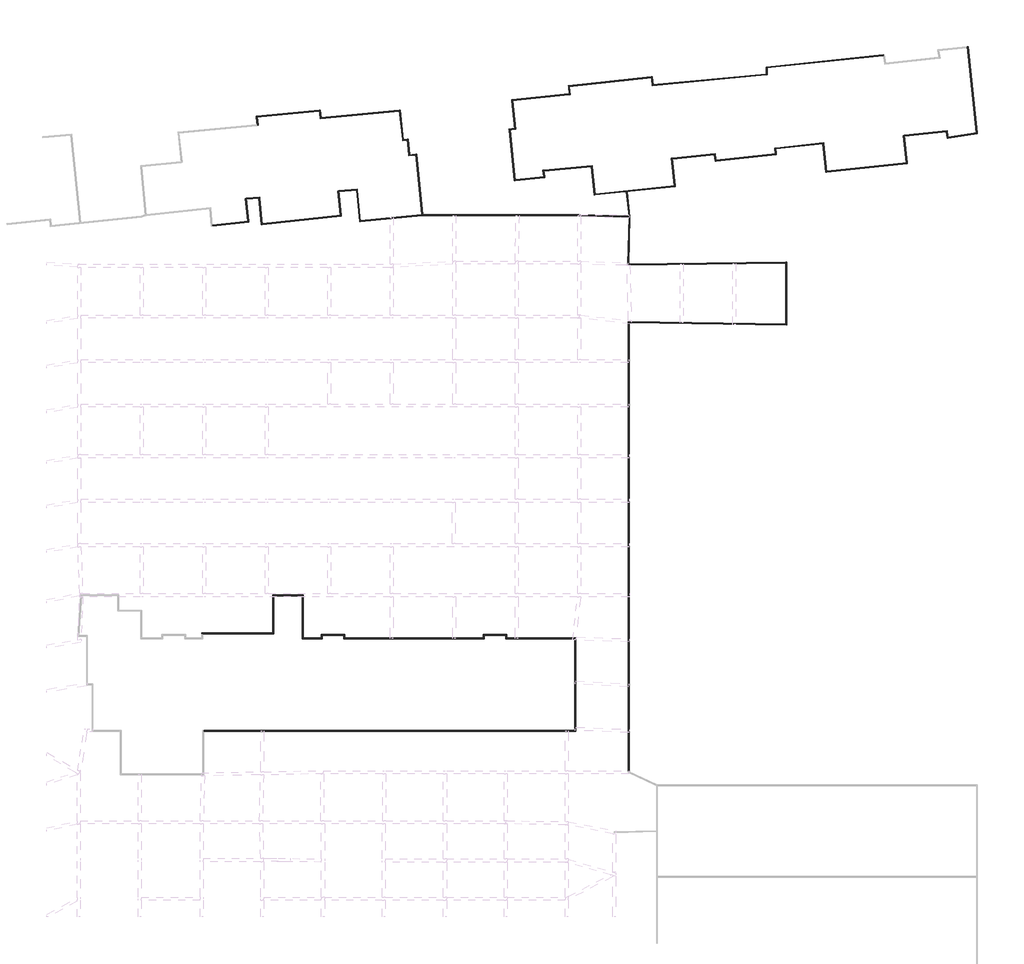
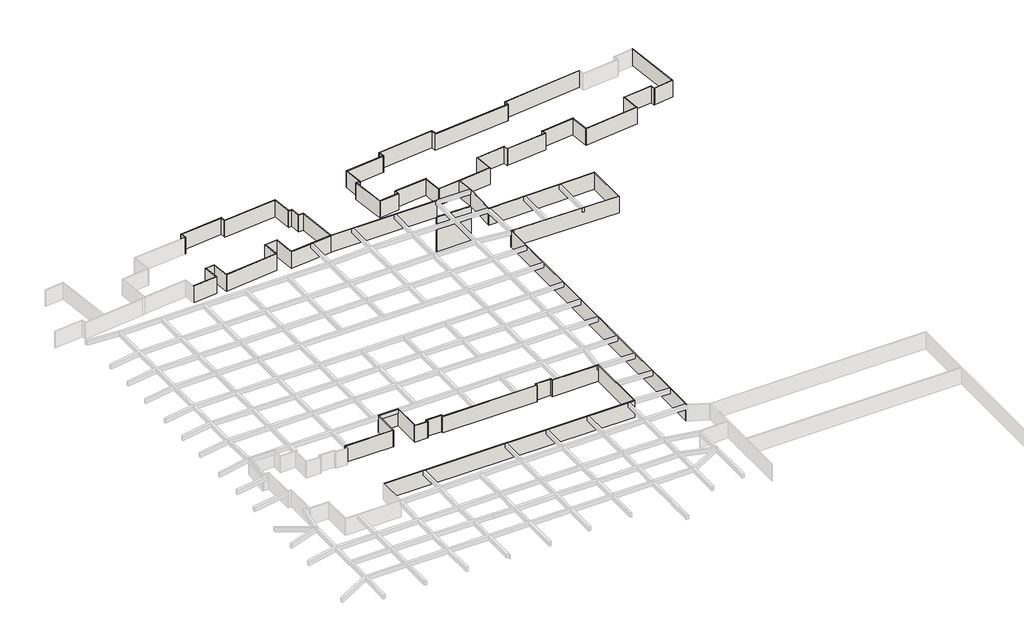
# One storey, part 7 of 20: 70 walls.
"""IFC4 building model written with IfcOpenShell, lengths in millimetres."""

from ifc_helpers import new_model, si_unit, frame, origin, origin_with_axes, place, context, project, spatial, polyline, outline, extrude, faceted_brep, element, save

model = new_model("IFC4")

# Units and contexts
model_context = context("Model", 3, world=origin())
ifc_project = project(units=[si_unit("LENGTHUNIT", "METRE", prefix="MILLI")], contexts=[model_context])

# Site, building, storey
site = spatial("IfcSite", under=ifc_project)
building = spatial("IfcBuilding", under=site)
storey = spatial("IfcBuildingStorey", under=building, Name="户型图", Elevation=0.0)

# Walls
placement = place(None, origin())
element("IfcWall", 1, ObjectType="所有墙体", at=placement, inside=storey, context=model_context, shape_type="SweptSolid", body=[
    extrude(outline(polyline([(179359.7688515, 185330.8967461), (179359.7688515, 127752.6972626), (179239.7688515, 127808.6541816), (179239.7688515, 185332.6895961), (179359.7688515, 185330.8967461)])), origin_with_axes(), (0.0, 0.0, 1.0), 3300.0),
])
element("IfcWall", 2, ObjectType="所有墙体", at=placement, inside=storey, context=model_context, shape_type="Brep", body=[
    faceted_brep([(179239.7688515, 185332.6895961, 0.0), (179359.7688515, 185330.8967461, 0.0), (199560.0, 185029.0968789, 0.0), (199560.0, 185029.0968789, 3300.0), (179359.7688515, 185330.8967461, 3300.0), (179239.7688515, 185332.6895961, 3300.0), (179239.7688515, 185452.7029883, 0.0), (179239.7688515, 185452.7029883, 3300.0), (199560.0, 185149.1102711, 3300.0), (199560.0, 185149.1102711, 0.0)], [[[0, 1, 2, 3, 4, 5]], [[6, 7, 8, 9]], [[2, 1, 0, 6, 9]], [[5, 4, 3, 8, 7]], [[0, 5, 7, 6]], [[3, 2, 9, 8]]]),
])
element("IfcWall", 3, ObjectType="所有墙体", at=placement, inside=storey, context=model_context, shape_type="Brep", body=[
    faceted_brep([(199560.0, 185149.1102711, 0.0), (199560.0, 193050.6703703, 0.0), (199560.0, 193050.6703703, 3300.0), (199560.0, 185149.1102711, 3300.0), (199440.0, 185150.9031211, 0.0), (199440.0, 185150.9031211, 3300.0), (199440.0, 192929.3296297, 3300.0), (199440.0, 193049.3370369, 3300.0), (199440.0, 193049.3370369, 0.0), (199440.0, 192929.3296297, 0.0)], [[[0, 1, 2, 3]], [[4, 5, 6, 7, 8, 9]], [[1, 0, 4, 9, 8]], [[3, 2, 7, 6, 5]], [[2, 1, 8, 7]], [[0, 3, 5, 4]]]),
])
element("IfcWall", 4, ObjectType="所有墙体", at=placement, inside=storey, context=model_context, shape_type="Brep", body=[
    faceted_brep([(199440.0, 193049.3370369, 0.0), (179311.5042041, 192825.6870836, 0.0), (179191.4355527, 192824.3529875, 0.0), (179191.4355527, 192824.3529875, 3300.0), (179311.5042041, 192825.6870836, 3300.0), (199440.0, 193049.3370369, 3300.0), (199440.0, 192929.3296297, 0.0), (199440.0, 192929.3296297, 3300.0), (179188.4957959, 192704.3129164, 3300.0), (179188.4957959, 192704.3129164, 0.0)], [[[0, 1, 2, 3, 4, 5]], [[6, 7, 8, 9]], [[2, 1, 0, 6, 9]], [[5, 4, 3, 8, 7]], [[0, 5, 7, 6]], [[3, 2, 9, 8]]]),
])
element("IfcWall", 5, ObjectType="所有墙体", at=placement, inside=storey, context=model_context, shape_type="SweptSolid", body=[
    extrude(outline(polyline([(179460.0770452, 198892.4114303), (179311.5042041, 192825.6870836), (179191.4355527, 192824.3529875), (179339.9229548, 198887.5885697), (179460.0770452, 198892.4114303)])), origin_with_axes(), (0.0, 0.0, 1.0), 3300.0),
])
element("IfcWall", 6, ObjectType="所有墙体", at=placement, inside=storey, context=model_context, shape_type="SweptSolid", body=[
    extrude(outline(polyline([(179120.9990927, 202118.5226488), (179460.0770452, 198892.4114303), (179339.9229548, 198887.5885697), (179001.6564653, 202105.9792332), (179120.9990927, 202118.5226488)])), origin_with_axes(), (0.0, 0.0, 1.0), 3300.0),
])
element("IfcWall", 7, ObjectType="所有墙体", at=placement, inside=storey, context=model_context, shape_type="Brep", body=[
    faceted_brep([(175009.081088, 201686.3426514, 0.0), (179001.6564653, 202105.9792332, 0.0), (179120.9990927, 202118.5226488, 0.0), (185275.013613, 202765.3356388, 0.0), (185275.013613, 202765.3356388, 3300.0), (179120.9990927, 202118.5226488, 3300.0), (179001.6564653, 202105.9792332, 3300.0), (175009.081088, 201686.3426514, 3300.0), (174996.5376724, 201805.6852789, 0.0), (174996.5376724, 201805.6852789, 3300.0), (185143.1275699, 202872.1348506, 3300.0), (185262.4701974, 202884.6782662, 3300.0), (185262.4701974, 202884.6782662, 0.0), (185143.1275699, 202872.1348506, 0.0)], [[[0, 1, 2, 3, 4, 5, 6, 7]], [[8, 9, 10, 11, 12, 13]], [[3, 2, 1, 0, 8, 13, 12]], [[7, 6, 5, 4, 11, 10, 9]], [[4, 3, 12, 11]], [[0, 7, 9, 8]]]),
])
element("IfcWall", 8, ObjectType="所有墙体", at=placement, inside=storey, context=model_context, shape_type="Brep", body=[
    faceted_brep([(185262.4701974, 202884.6782662, 0.0), (184906.1157461, 206275.1643906, 0.0), (184893.5723305, 206394.5070181, 0.0), (184893.5723305, 206394.5070181, 3300.0), (184906.1157461, 206275.1643906, 3300.0), (185262.4701974, 202884.6782662, 3300.0), (185143.1275699, 202872.1348506, 0.0), (185143.1275699, 202872.1348506, 3300.0), (184774.229703, 206381.9636025, 3300.0), (184774.229703, 206381.9636025, 0.0)], [[[0, 1, 2, 3, 4, 5]], [[6, 7, 8, 9]], [[2, 1, 0, 6, 9]], [[5, 4, 3, 8, 7]], [[0, 5, 7, 6]], [[3, 2, 9, 8]]]),
])
element("IfcWall", 9, ObjectType="所有墙体", at=placement, inside=storey, context=model_context, shape_type="Brep", body=[
    faceted_brep([(184906.1157461, 206275.1643906, 0.0), (190280.8750728, 206840.0743594, 0.0), (190400.2177003, 206852.617775, 0.0), (190400.2177003, 206852.617775, 3300.0), (190280.8750728, 206840.0743594, 3300.0), (184906.1157461, 206275.1643906, 3300.0), (184893.5723305, 206394.5070181, 0.0), (184893.5723305, 206394.5070181, 3300.0), (190387.6742847, 206971.9604024, 3300.0), (190387.6742847, 206971.9604024, 0.0)], [[[0, 1, 2, 3, 4, 5]], [[6, 7, 8, 9]], [[2, 1, 0, 6, 9]], [[5, 4, 3, 8, 7]], [[0, 5, 7, 6]], [[3, 2, 9, 8]]]),
])
element("IfcWall", 10, ObjectType="所有墙体", at=placement, inside=storey, context=model_context, shape_type="Brep", body=[
    faceted_brep([(190280.8750728, 206840.0743594, 0.0), (190368.4732423, 206006.6334497, 0.0), (190368.4732423, 206006.6334497, 3300.0), (190280.8750728, 206840.0743594, 3300.0), (190400.2177003, 206852.617775, 0.0), (190400.2177003, 206852.617775, 3300.0), (190475.2724541, 206138.5194927, 3300.0), (190487.8158697, 206019.1768653, 3300.0), (190487.8158697, 206019.1768653, 0.0), (190475.2724541, 206138.5194927, 0.0)], [[[0, 1, 2, 3]], [[4, 5, 6, 7, 8, 9]], [[1, 0, 4, 9, 8]], [[3, 2, 7, 6, 5]], [[0, 3, 5, 4]], [[2, 1, 8, 7]]]),
])
element("IfcWall", 11, ObjectType="所有墙体", at=placement, inside=storey, context=model_context, shape_type="Brep", body=[
    faceted_brep([(190487.8158697, 206019.1768653, 0.0), (198188.6858964, 206828.5709203, 0.0), (198188.6858964, 206828.5709203, 3300.0), (190487.8158697, 206019.1768653, 3300.0), (190475.2724541, 206138.5194927, 0.0), (190475.2724541, 206138.5194927, 3300.0), (198056.7998534, 206935.3701322, 3300.0), (198176.1424808, 206947.9135478, 3300.0), (198176.1424808, 206947.9135478, 0.0), (198056.7998534, 206935.3701322, 0.0)], [[[0, 1, 2, 3]], [[4, 5, 6, 7, 8, 9]], [[1, 0, 4, 9, 8]], [[3, 2, 7, 6, 5]], [[0, 3, 5, 4]], [[2, 1, 8, 7]]]),
])
element("IfcWall", 12, ObjectType="所有墙体", at=placement, inside=storey, context=model_context, shape_type="Brep", body=[
    faceted_brep([(198176.1424808, 206947.9135478, 0.0), (198110.6347971, 207571.1775256, 0.0), (198098.0913815, 207690.520153, 0.0), (198098.0913815, 207690.520153, 3300.0), (198110.6347971, 207571.1775256, 3300.0), (198176.1424808, 206947.9135478, 3300.0), (198056.7998534, 206935.3701322, 0.0), (198056.7998534, 206935.3701322, 3300.0), (197978.748754, 207677.9767374, 3300.0), (197978.748754, 207677.9767374, 0.0)], [[[0, 1, 2, 3, 4, 5]], [[6, 7, 8, 9]], [[2, 1, 0, 6, 9]], [[5, 4, 3, 8, 7]], [[0, 5, 7, 6]], [[3, 2, 9, 8]]]),
])
element("IfcWall", 13, ObjectType="所有墙体", at=placement, inside=storey, context=model_context, shape_type="Brep", body=[
    faceted_brep([(198110.6347971, 207571.1775256, 0.0), (204161.7596128, 208207.1763718, 0.0), (204281.1022402, 208219.7197874, 0.0), (204281.1022402, 208219.7197874, 3300.0), (204161.7596128, 208207.1763718, 3300.0), (198110.6347971, 207571.1775256, 3300.0), (198098.0913815, 207690.520153, 0.0), (198098.0913815, 207690.520153, 3300.0), (204268.5588247, 208339.0624149, 3300.0), (204268.5588247, 208339.0624149, 0.0)], [[[0, 1, 2, 3, 4, 5]], [[6, 7, 8, 9]], [[2, 1, 0, 6, 9]], [[5, 4, 3, 8, 7]], [[0, 5, 7, 6]], [[3, 2, 9, 8]]]),
])
element("IfcWall", 14, ObjectType="所有墙体", at=placement, inside=storey, context=model_context, shape_type="Brep", body=[
    faceted_brep([(204161.7596128, 208207.1763718, 0.0), (204542.5743461, 204583.9662099, 0.0), (204542.5743461, 204583.9662099, 3300.0), (204161.7596128, 208207.1763718, 3300.0), (204281.1022402, 208219.7197874, 0.0), (204281.1022402, 208219.7197874, 3300.0), (204649.3735579, 204715.8522529, 3300.0), (204661.9169735, 204596.5096255, 3300.0), (204661.9169735, 204596.5096255, 0.0), (204649.3735579, 204715.8522529, 0.0)], [[[0, 1, 2, 3]], [[4, 5, 6, 7, 8, 9]], [[1, 0, 4, 9, 8]], [[3, 2, 7, 6, 5]], [[0, 3, 5, 4]], [[2, 1, 8, 7]]]),
])
element("IfcWall", 15, ObjectType="所有墙体", at=placement, inside=storey, context=model_context, shape_type="Brep", body=[
    faceted_brep([(204661.9169735, 204596.5096255, 0.0), (214978.0466758, 205680.7785487, 0.0), (214978.0466758, 205680.7785487, 3300.0), (204661.9169735, 204596.5096255, 3300.0), (204649.3735579, 204715.8522529, 0.0), (204649.3735579, 204715.8522529, 3300.0), (214846.1606327, 205787.5777606, 3300.0), (214965.5032602, 205800.1211762, 3300.0), (214965.5032602, 205800.1211762, 0.0), (214846.1606327, 205787.5777606, 0.0)], [[[0, 1, 2, 3]], [[4, 5, 6, 7, 8, 9]], [[1, 0, 4, 9, 8]], [[3, 2, 7, 6, 5]], [[0, 3, 5, 4]], [[2, 1, 8, 7]]]),
])
element("IfcWall", 16, ObjectType="所有墙体", at=placement, inside=storey, context=model_context, shape_type="Brep", body=[
    faceted_brep([(214965.5032602, 205800.1211762, 0.0), (214609.1847922, 209190.2649423, 0.0), (214596.6413766, 209309.6075698, 0.0), (214596.6413766, 209309.6075698, 3300.0), (214609.1847922, 209190.2649423, 3300.0), (214965.5032602, 205800.1211762, 3300.0), (214846.1606327, 205787.5777606, 0.0), (214846.1606327, 205787.5777606, 3300.0), (214477.2987492, 209297.0641542, 3300.0), (214477.2987492, 209297.0641542, 0.0)], [[[0, 1, 2, 3, 4, 5]], [[6, 7, 8, 9]], [[2, 1, 0, 6, 9]], [[5, 4, 3, 8, 7]], [[0, 5, 7, 6]], [[3, 2, 9, 8]]]),
])
element("IfcWall", 17, ObjectType="所有墙体", at=placement, inside=storey, context=model_context, shape_type="Brep", body=[
    faceted_brep([(214609.1847922, 209190.2649423, 0.0), (219982.9732093, 209755.0728644, 0.0), (220102.3158367, 209767.61628, 0.0), (220102.3158367, 209767.61628, 3300.0), (219982.9732093, 209755.0728644, 3300.0), (214609.1847922, 209190.2649423, 3300.0), (214596.6413766, 209309.6075698, 0.0), (214596.6413766, 209309.6075698, 3300.0), (220089.7724211, 209886.9589074, 3300.0), (220089.7724211, 209886.9589074, 0.0)], [[[0, 1, 2, 3, 4, 5]], [[6, 7, 8, 9]], [[2, 1, 0, 6, 9]], [[5, 4, 3, 8, 7]], [[0, 5, 7, 6]], [[3, 2, 9, 8]]]),
])
element("IfcWall", 18, ObjectType="所有墙体", at=placement, inside=storey, context=model_context, shape_type="Brep", body=[
    faceted_brep([(219982.9732093, 209755.0728644, 0.0), (220070.8035215, 208919.4232641, 0.0), (220070.8035215, 208919.4232641, 3300.0), (219982.9732093, 209755.0728644, 3300.0), (220102.3158367, 209767.61628, 0.0), (220102.3158367, 209767.61628, 3300.0), (220176.9281469, 209057.7275686, 3300.0), (220189.4887764, 208938.2211617, 3300.0), (220189.4887764, 208938.2211617, 0.0), (220176.9281469, 209057.7275686, 0.0)], [[[0, 1, 2, 3]], [[4, 5, 6, 7, 8, 9]], [[1, 0, 4, 9, 8]], [[3, 2, 7, 6, 5]], [[0, 3, 5, 4]], [[2, 1, 8, 7]]]),
])
element("IfcWall", 19, ObjectType="所有墙体", at=placement, inside=storey, context=model_context, shape_type="Brep", body=[
    faceted_brep([(220189.4887764, 208938.2211617, 0.0), (223943.6146969, 209532.8162946, 0.0), (223943.6146969, 209532.8162946, 3300.0), (220189.4887764, 208938.2211617, 3300.0), (220176.9281469, 209057.7275686, 0.0), (220176.9281469, 209057.7275686, 3300.0), (223812.3688125, 209633.5248037, 3300.0), (223931.0540674, 209652.3227014, 3300.0), (223931.0540674, 209652.3227014, 0.0), (223812.3688125, 209633.5248037, 0.0)], [[[0, 1, 2, 3]], [[4, 5, 6, 7, 8, 9]], [[1, 0, 4, 9, 8]], [[3, 2, 7, 6, 5]], [[0, 3, 5, 4]], [[2, 1, 8, 7]]]),
])
element("IfcWall", 20, ObjectType="所有墙体", at=placement, inside=storey, context=model_context, shape_type="Brep", body=[
    faceted_brep([(223931.0540674, 209652.3227014, 0.0), (222771.1254183, 220688.3066092, 0.0), (222771.1254183, 220688.3066092, 3300.0), (223931.0540674, 209652.3227014, 3300.0), (223812.3688125, 209633.5248037, 0.0), (223812.3688125, 209633.5248037, 3300.0), (222664.3262065, 220556.4205662, 3300.0), (222651.7827909, 220675.7631937, 3300.0), (222651.7827909, 220675.7631937, 0.0), (222664.3262065, 220556.4205662, 0.0)], [[[0, 1, 2, 3]], [[4, 5, 6, 7, 8, 9]], [[1, 0, 4, 9, 8]], [[3, 2, 7, 6, 5]], [[0, 3, 5, 4]], [[2, 1, 8, 7]]]),
])
element("IfcWall", 21, ObjectType="所有墙体", at=placement, inside=storey, context=model_context, shape_type="Brep", body=[
    faceted_brep([(211896.3577151, 219645.7354926, 0.0), (196892.6398704, 218068.7812024, 0.0), (196892.6398704, 218068.7812024, 3300.0), (211896.3577151, 219645.7354926, 3300.0), (211915.1556128, 219527.0502378, 0.0), (211915.1556128, 219527.0502378, 3300.0), (197012.6398704, 217960.7327171, 3300.0), (196892.6398704, 217948.1202089, 3300.0), (196892.6398704, 217948.1202089, 0.0), (197012.6398704, 217960.7327171, 0.0)], [[[0, 1, 2, 3]], [[4, 5, 6, 7, 8, 9]], [[1, 0, 4, 9, 8]], [[3, 2, 7, 6, 5]], [[0, 3, 5, 4]], [[2, 1, 8, 7]]]),
])
element("IfcWall", 22, ObjectType="所有墙体", at=placement, inside=storey, context=model_context, shape_type="Brep", body=[
    faceted_brep([(196892.6398704, 217948.1202089, 0.0), (196892.6398704, 217169.3650376, 0.0), (196892.6398704, 217048.832647, 0.0), (196892.6398704, 217048.832647, 3300.0), (196892.6398704, 217169.3650376, 3300.0), (196892.6398704, 217948.1202089, 3300.0), (197012.6398704, 217960.7327171, 0.0), (197012.6398704, 217960.7327171, 3300.0), (197012.6398704, 217060.148882, 3300.0), (197012.6398704, 217060.148882, 0.0)], [[[0, 1, 2, 3, 4, 5]], [[6, 7, 8, 9]], [[2, 1, 0, 6, 9]], [[5, 4, 3, 8, 7]], [[0, 5, 7, 6]], [[3, 2, 9, 8]]]),
])
element("IfcWall", 23, ObjectType="所有墙体", at=placement, inside=storey, context=model_context, shape_type="Brep", body=[
    faceted_brep([(196892.6398704, 217169.3650376, 0.0), (182438.466331, 215806.308175, 0.0), (182318.9895359, 215795.0412793, 0.0), (182318.9895359, 215795.0412793, 3300.0), (182438.466331, 215806.308175, 3300.0), (196892.6398704, 217169.3650376, 3300.0), (196892.6398704, 217048.832647, 0.0), (196892.6398704, 217048.832647, 3300.0), (182331.533669, 215675.691825, 3300.0), (182331.533669, 215675.691825, 0.0)], [[[0, 1, 2, 3, 4, 5]], [[6, 7, 8, 9]], [[2, 1, 0, 6, 9]], [[5, 4, 3, 8, 7]], [[0, 5, 7, 6]], [[3, 2, 9, 8]]]),
])
element("IfcWall", 24, ObjectType="所有墙体", at=placement, inside=storey, context=model_context, shape_type="Brep", body=[
    faceted_brep([(182438.466331, 215806.308175, 0.0), (182333.8711427, 216801.4649169, 0.0), (182333.8711427, 216801.4649169, 3300.0), (182438.466331, 215806.308175, 3300.0), (182318.9895359, 215795.0412793, 0.0), (182318.9895359, 215795.0412793, 3300.0), (182227.0719308, 216669.5788739, 3300.0), (182214.5285152, 216788.9215013, 3300.0), (182214.5285152, 216788.9215013, 0.0), (182227.0719308, 216669.5788739, 0.0)], [[[0, 1, 2, 3]], [[4, 5, 6, 7, 8, 9]], [[1, 0, 4, 9, 8]], [[3, 2, 7, 6, 5]], [[0, 3, 5, 4]], [[2, 1, 8, 7]]]),
])
element("IfcWall", 25, ObjectType="所有墙体", at=placement, inside=storey, context=model_context, shape_type="Brep", body=[
    faceted_brep([(182214.5285152, 216788.9215013, 0.0), (171581.168922, 215671.3103729, 0.0), (171581.168922, 215671.3103729, 3300.0), (182214.5285152, 216788.9215013, 3300.0), (182227.0719308, 216669.5788739, 0.0), (182227.0719308, 216669.5788739, 3300.0), (171713.054965, 215564.5111611, 3300.0), (171593.7123376, 215551.9677455, 3300.0), (171593.7123376, 215551.9677455, 0.0), (171713.054965, 215564.5111611, 0.0)], [[[0, 1, 2, 3]], [[4, 5, 6, 7, 8, 9]], [[1, 0, 4, 9, 8]], [[3, 2, 7, 6, 5]], [[0, 3, 5, 4]], [[2, 1, 8, 7]]]),
])
element("IfcWall", 26, ObjectType="所有墙体", at=placement, inside=storey, context=model_context, shape_type="Brep", body=[
    faceted_brep([(171593.7123376, 215551.9677455, 0.0), (171690.7043845, 214629.150062, 0.0), (171703.2478001, 214509.8074345, 0.0), (171703.2478001, 214509.8074345, 3300.0), (171690.7043845, 214629.150062, 3300.0), (171593.7123376, 215551.9677455, 3300.0), (171713.054965, 215564.5111611, 0.0), (171713.054965, 215564.5111611, 3300.0), (171822.5904275, 214522.3508501, 3300.0), (171822.5904275, 214522.3508501, 0.0)], [[[0, 1, 2, 3, 4, 5]], [[6, 7, 8, 9]], [[2, 1, 0, 6, 9]], [[5, 4, 3, 8, 7]], [[0, 5, 7, 6]], [[3, 2, 9, 8]]]),
])
element("IfcWall", 27, ObjectType="所有墙体", at=placement, inside=storey, context=model_context, shape_type="Brep", body=[
    faceted_brep([(171690.7043845, 214629.150062, 0.0), (164300.405986, 213852.3984004, 0.0), (164300.405986, 213852.3984004, 3300.0), (171690.7043845, 214629.150062, 3300.0), (171703.2478001, 214509.8074345, 0.0), (171703.2478001, 214509.8074345, 3300.0), (164432.2920291, 213745.5991886, 3300.0), (164312.9494016, 213733.055773, 3300.0), (164312.9494016, 213733.055773, 0.0), (164432.2920291, 213745.5991886, 0.0)], [[[0, 1, 2, 3]], [[4, 5, 6, 7, 8, 9]], [[1, 0, 4, 9, 8]], [[3, 2, 7, 6, 5]], [[0, 3, 5, 4]], [[2, 1, 8, 7]]]),
])
element("IfcWall", 28, ObjectType="所有墙体", at=placement, inside=storey, context=model_context, shape_type="Brep", body=[
    faceted_brep([(164312.9494016, 213733.055773, 0.0), (164684.8655737, 210194.5097657, 0.0), (164697.4089893, 210075.1671382, 0.0), (164697.4089893, 210075.1671382, 3300.0), (164684.8655737, 210194.5097657, 3300.0), (164312.9494016, 213733.055773, 3300.0), (164432.2920291, 213745.5991886, 0.0), (164432.2920291, 213745.5991886, 3300.0), (164816.7516167, 210087.7105538, 3300.0), (164816.7516167, 210087.7105538, 0.0)], [[[0, 1, 2, 3, 4, 5]], [[6, 7, 8, 9]], [[2, 1, 0, 6, 9]], [[5, 4, 3, 8, 7]], [[0, 5, 7, 6]], [[3, 2, 9, 8]]]),
])
element("IfcWall", 29, ObjectType="所有墙体", at=placement, inside=storey, context=model_context, shape_type="Brep", body=[
    faceted_brep([(164684.8655737, 210194.5097657, 0.0), (163969.8374545, 210119.357282, 0.0), (163969.8374545, 210119.357282, 3300.0), (164684.8655737, 210194.5097657, 3300.0), (164697.4089893, 210075.1671382, 0.0), (164697.4089893, 210075.1671382, 3300.0), (164101.7234975, 210012.5580702, 3300.0), (163982.3808701, 210000.0146546, 3300.0), (163982.3808701, 210000.0146546, 0.0), (164101.7234975, 210012.5580702, 0.0)], [[[0, 1, 2, 3]], [[4, 5, 6, 7, 8, 9]], [[1, 0, 4, 9, 8]], [[3, 2, 7, 6, 5]], [[0, 3, 5, 4]], [[2, 1, 8, 7]]]),
])
element("IfcWall", 30, ObjectType="所有墙体", at=placement, inside=storey, context=model_context, shape_type="Brep", body=[
    faceted_brep([(163982.3808701, 210000.0146546, 0.0), (164664.446564, 203510.5930613, 0.0), (164664.446564, 203510.5930613, 3300.0), (163982.3808701, 210000.0146546, 3300.0), (164101.7234975, 210012.5580702, 0.0), (164101.7234975, 210012.5580702, 3300.0), (164771.2457758, 203642.4791043, 3300.0), (164783.7891914, 203523.1364769, 3300.0), (164783.7891914, 203523.1364769, 0.0), (164771.2457758, 203642.4791043, 0.0)], [[[0, 1, 2, 3]], [[4, 5, 6, 7, 8, 9]], [[1, 0, 4, 9, 8]], [[3, 2, 7, 6, 5]], [[0, 3, 5, 4]], [[2, 1, 8, 7]]]),
])
element("IfcWall", 31, ObjectType="所有墙体", at=placement, inside=storey, context=model_context, shape_type="Brep", body=[
    faceted_brep([(164783.7891914, 203523.1364769, 0.0), (168536.3797426, 203917.549637, 0.0), (168536.3797426, 203917.549637, 3300.0), (164783.7891914, 203523.1364769, 3300.0), (164771.2457758, 203642.4791043, 0.0), (164771.2457758, 203642.4791043, 3300.0), (168404.4936996, 204024.3488489, 3300.0), (168523.836327, 204036.8922645, 3300.0), (168523.836327, 204036.8922645, 0.0), (168404.4936996, 204024.3488489, 0.0)], [[[0, 1, 2, 3]], [[4, 5, 6, 7, 8, 9]], [[1, 0, 4, 9, 8]], [[3, 2, 7, 6, 5]], [[0, 3, 5, 4]], [[2, 1, 8, 7]]]),
])
element("IfcWall", 32, ObjectType="所有墙体", at=placement, inside=storey, context=model_context, shape_type="Brep", body=[
    faceted_brep([(168523.836327, 204036.8922645, 0.0), (168453.0383983, 204710.4895608, 0.0), (168440.4942645, 204829.8390215, 0.0), (168440.4942645, 204829.8390215, 3300.0), (168453.0383983, 204710.4895608, 3300.0), (168523.836327, 204036.8922645, 3300.0), (168404.4936996, 204024.3488489, 0.0), (168404.4936996, 204024.3488489, 3300.0), (168321.0174056, 204818.5727331, 3300.0), (168321.0174056, 204818.5727331, 0.0)], [[[0, 1, 2, 3, 4, 5]], [[6, 7, 8, 9]], [[2, 1, 0, 6, 9]], [[5, 4, 3, 8, 7]], [[0, 5, 7, 6]], [[3, 2, 9, 8]]]),
])
element("IfcWall", 33, ObjectType="所有墙体", at=placement, inside=storey, context=model_context, shape_type="Brep", body=[
    faceted_brep([(168453.0383983, 204710.4895608, 0.0), (174510.5336374, 205281.6921254, 0.0), (174630.0104964, 205292.9584138, 0.0), (174630.0104964, 205292.9584138, 3300.0), (174510.5336374, 205281.6921254, 3300.0), (168453.0383983, 204710.4895608, 3300.0), (168440.4942645, 204829.8390215, 0.0), (168440.4942645, 204829.8390215, 3300.0), (174617.4663626, 205412.3078746, 3300.0), (174617.4663626, 205412.3078746, 0.0)], [[[0, 1, 2, 3, 4, 5]], [[6, 7, 8, 9]], [[2, 1, 0, 6, 9]], [[5, 4, 3, 8, 7]], [[0, 5, 7, 6]], [[3, 2, 9, 8]]]),
])
element("IfcWall", 34, ObjectType="所有墙体", at=placement, inside=storey, context=model_context, shape_type="Brep", body=[
    faceted_brep([(174510.5336374, 205281.6921254, 0.0), (174889.7384605, 201673.7992358, 0.0), (174889.7384605, 201673.7992358, 3300.0), (174510.5336374, 205281.6921254, 3300.0), (174630.0104964, 205292.9584138, 0.0), (174630.0104964, 205292.9584138, 3300.0), (174996.5376724, 201805.6852789, 3300.0), (175009.081088, 201686.3426514, 3300.0), (175009.081088, 201686.3426514, 0.0), (174996.5376724, 201805.6852789, 0.0)], [[[0, 1, 2, 3]], [[4, 5, 6, 7, 8, 9]], [[1, 0, 4, 9, 8]], [[3, 2, 7, 6, 5]], [[0, 3, 5, 4]], [[2, 1, 8, 7]]]),
])
element("IfcWall", 35, ObjectType="所有墙体", at=placement, inside=storey, context=model_context, shape_type="Brep", body=[
    faceted_brep([(152798.3916431, 199007.0, 0.0), (172953.0, 199007.0, 0.0), (172953.0, 199007.0, 3300.0), (152798.3916431, 199007.0, 3300.0), (152787.0760242, 199127.0, 0.0), (152787.0760242, 199127.0, 3300.0), (152907.6083569, 199127.0, 3300.0), (172953.0, 199127.0, 3300.0), (172953.0, 199127.0, 0.0), (152907.6083569, 199127.0, 0.0)], [[[0, 1, 2, 3]], [[4, 5, 6, 7, 8, 9]], [[1, 0, 4, 9, 8]], [[2, 1, 8, 7]], [[3, 2, 7, 6, 5]], [[0, 3, 5, 4]]]),
])
element("IfcWall", 36, ObjectType="所有墙体", at=placement, inside=storey, context=model_context, shape_type="Brep", body=[
    faceted_brep([(172953.0, 199127.0, 0.0), (152907.6083569, 199127.0, 0.0), (152787.0760242, 199127.0, 0.0), (152787.0760242, 199127.0, 3300.0), (152907.6083569, 199127.0, 3300.0), (172953.0, 199127.0, 3300.0), (172953.0, 199007.0, 0.0), (172953.0, 199007.0, 3300.0), (152798.3916431, 199007.0, 3300.0), (152798.3916431, 199007.0, 0.0)], [[[0, 1, 2, 3, 4, 5]], [[6, 7, 8, 9]], [[2, 1, 0, 6, 9]], [[5, 4, 3, 8, 7]], [[0, 5, 7, 6]], [[3, 2, 9, 8]]]),
])
element("IfcWall", 37, ObjectType="所有墙体", at=placement, inside=storey, context=model_context, shape_type="Brep", body=[
    faceted_brep([(152907.6083569, 199127.0, 0.0), (152174.8353707, 206897.9190224, 0.0), (152174.8353707, 206897.9190224, 3300.0), (152907.6083569, 199127.0, 3300.0), (152787.0760242, 199127.0, 0.0), (152787.0760242, 199127.0, 3300.0), (152066.6309957, 206767.1833607, 3300.0), (152055.3653523, 206886.6533791, 3300.0), (152055.3653523, 206886.6533791, 0.0), (152066.6309957, 206767.1833607, 0.0)], [[[0, 1, 2, 3]], [[4, 5, 6, 7, 8, 9]], [[1, 0, 4, 9, 8]], [[3, 2, 7, 6, 5]], [[0, 3, 5, 4]], [[2, 1, 8, 7]]]),
])
element("IfcWall", 38, ObjectType="所有墙体", at=placement, inside=storey, context=model_context, shape_type="Brep", body=[
    faceted_brep([(152055.3653523, 206886.6533791, 0.0), (151247.154558, 206810.4416677, 0.0), (151127.6776991, 206799.1753794, 0.0), (151127.6776991, 206799.1753794, 3300.0), (151247.154558, 206810.4416677, 3300.0), (152055.3653523, 206886.6533791, 3300.0), (152066.6309957, 206767.1833607, 0.0), (152066.6309957, 206767.1833607, 3300.0), (151140.2218329, 206679.8259186, 3300.0), (151140.2218329, 206679.8259186, 0.0)], [[[0, 1, 2, 3, 4, 5]], [[6, 7, 8, 9]], [[2, 1, 0, 6, 9]], [[5, 4, 3, 8, 7]], [[0, 5, 7, 6]], [[3, 2, 9, 8]]]),
])
element("IfcWall", 39, ObjectType="所有墙体", at=placement, inside=storey, context=model_context, shape_type="Brep", body=[
    faceted_brep([(151247.154558, 206810.4416677, 0.0), (151038.0308748, 208800.1206054, 0.0), (151038.0308748, 208800.1206054, 3300.0), (151247.154558, 206810.4416677, 3300.0), (151127.6776991, 206799.1753794, 0.0), (151127.6776991, 206799.1753794, 3300.0), (150931.231663, 208668.2345624, 3300.0), (150918.6882474, 208787.5771898, 3300.0), (150918.6882474, 208787.5771898, 0.0), (150931.231663, 208668.2345624, 0.0)], [[[0, 1, 2, 3]], [[4, 5, 6, 7, 8, 9]], [[1, 0, 4, 9, 8]], [[3, 2, 7, 6, 5]], [[0, 3, 5, 4]], [[2, 1, 8, 7]]]),
])
element("IfcWall", 40, ObjectType="所有墙体", at=placement, inside=storey, context=model_context, shape_type="Brep", body=[
    faceted_brep([(150918.6882474, 208787.5771898, 0.0), (150455.4053887, 208738.8841993, 0.0), (150336.0627612, 208726.3407837, 0.0), (150336.0627612, 208726.3407837, 3300.0), (150455.4053887, 208738.8841993, 3300.0), (150918.6882474, 208787.5771898, 3300.0), (150931.231663, 208668.2345624, 0.0), (150931.231663, 208668.2345624, 3300.0), (150348.6061768, 208606.9981562, 3300.0), (150348.6061768, 208606.9981562, 0.0)], [[[0, 1, 2, 3, 4, 5]], [[6, 7, 8, 9]], [[2, 1, 0, 6, 9]], [[5, 4, 3, 8, 7]], [[0, 5, 7, 6]], [[3, 2, 9, 8]]]),
])
element("IfcWall", 41, ObjectType="所有墙体", at=placement, inside=storey, context=model_context, shape_type="Brep", body=[
    faceted_brep([(150455.4053887, 208738.8841993, 0.0), (150058.014302, 212519.807829, 0.0), (150058.014302, 212519.807829, 3300.0), (150455.4053887, 208738.8841993, 3300.0), (150336.0627612, 208726.3407837, 0.0), (150336.0627612, 208726.3407837, 3300.0), (149951.0815768, 212389.1920799, 3300.0), (149938.537443, 212508.5415406, 3300.0), (149938.537443, 212508.5415406, 0.0), (149951.0815768, 212389.1920799, 0.0)], [[[0, 1, 2, 3]], [[4, 5, 6, 7, 8, 9]], [[1, 0, 4, 9, 8]], [[3, 2, 7, 6, 5]], [[0, 3, 5, 4]], [[2, 1, 8, 7]]]),
])
element("IfcWall", 42, ObjectType="所有墙体", at=placement, inside=storey, context=model_context, shape_type="Brep", body=[
    faceted_brep([(149938.537443, 212508.5415406, 0.0), (139903.0627437, 211562.2281455, 0.0), (139783.5858848, 211550.9618571, 0.0), (139783.5858848, 211550.9618571, 3300.0), (139903.0627437, 211562.2281455, 3300.0), (149938.537443, 212508.5415406, 3300.0), (149951.0815768, 212389.1920799, 0.0), (149951.0815768, 212389.1920799, 3300.0), (139796.1300186, 211431.6123963, 3300.0), (139796.1300186, 211431.6123963, 0.0)], [[[0, 1, 2, 3, 4, 5]], [[6, 7, 8, 9]], [[2, 1, 0, 6, 9]], [[5, 4, 3, 8, 7]], [[0, 5, 7, 6]], [[3, 2, 9, 8]]]),
])
element("IfcWall", 43, ObjectType="所有墙体", at=placement, inside=storey, context=model_context, shape_type="Brep", body=[
    faceted_brep([(139903.0627437, 211562.2281455, 0.0), (139798.5342805, 212556.7500408, 0.0), (139798.5342805, 212556.7500408, 3300.0), (139903.0627437, 211562.2281455, 3300.0), (139783.5858848, 211550.9618571, 0.0), (139783.5858848, 211550.9618571, 3300.0), (139691.6015554, 212426.1342917, 3300.0), (139679.0574216, 212545.4837524, 3300.0), (139679.0574216, 212545.4837524, 0.0), (139691.6015554, 212426.1342917, 0.0)], [[[0, 1, 2, 3]], [[4, 5, 6, 7, 8, 9]], [[1, 0, 4, 9, 8]], [[3, 2, 7, 6, 5]], [[0, 3, 5, 4]], [[2, 1, 8, 7]]]),
])
element("IfcWall", 44, ObjectType="所有墙体", at=placement, inside=storey, context=model_context, shape_type="Brep", body=[
    faceted_brep([(139679.0574216, 212545.4837524, 0.0), (131614.8311842, 211785.0528273, 0.0), (131614.8311842, 211785.0528273, 3300.0), (139679.0574216, 212545.4837524, 3300.0), (139691.6015554, 212426.1342917, 0.0), (139691.6015554, 212426.1342917, 3300.0), (131746.8521769, 211676.9696549, 3300.0), (131627.375318, 211665.7033665, 3300.0), (131627.375318, 211665.7033665, 0.0), (131746.8521769, 211676.9696549, 0.0)], [[[0, 1, 2, 3]], [[4, 5, 6, 7, 8, 9]], [[1, 0, 4, 9, 8]], [[3, 2, 7, 6, 5]], [[0, 3, 5, 4]], [[2, 1, 8, 7]]]),
])
element("IfcWall", 45, ObjectType="所有墙体", at=placement, inside=storey, context=model_context, shape_type="Brep", body=[
    faceted_brep([(131627.375318, 211665.7033665, 0.0), (131729.8124937, 210691.0787424, 0.0), (131742.3566275, 210571.7292816, 0.0), (131742.3566275, 210571.7292816, 3300.0), (131729.8124937, 210691.0787424, 3300.0), (131627.375318, 211665.7033665, 3300.0), (131746.8521769, 211676.9696549, 0.0), (131746.8521769, 211676.9696549, 3300.0), (131861.8334865, 210582.99557, 3300.0), (131861.8334865, 210582.99557, 0.0)], [[[0, 1, 2, 3, 4, 5]], [[6, 7, 8, 9]], [[2, 1, 0, 6, 9]], [[5, 4, 3, 8, 7]], [[0, 5, 7, 6]], [[3, 2, 9, 8]]]),
])
element("IfcWall", 46, ObjectType="所有墙体", at=placement, inside=storey, context=model_context, shape_type="Brep", body=[
    faceted_brep([(125983.7175969, 197708.3160064, 0.0), (130658.6056521, 198199.6665404, 0.0), (130658.6056521, 198199.6665404, 3300.0), (125983.7175969, 197708.3160064, 3300.0), (125972.4513085, 197827.7928654, 0.0), (125972.4513085, 197827.7928654, 3300.0), (130526.7196091, 198306.4657523, 3300.0), (130646.0622365, 198319.0091679, 3300.0), (130646.0622365, 198319.0091679, 0.0), (130526.7196091, 198306.4657523, 0.0)], [[[0, 1, 2, 3]], [[4, 5, 6, 7, 8, 9]], [[1, 0, 4, 9, 8]], [[3, 2, 7, 6, 5]], [[0, 3, 5, 4]], [[2, 1, 8, 7]]]),
])
element("IfcWall", 47, ObjectType="所有墙体", at=placement, inside=storey, context=model_context, shape_type="Brep", body=[
    faceted_brep([(130646.0622365, 198319.0091679, 0.0), (130352.1277628, 201115.6088769, 0.0), (130339.583629, 201234.9583376, 0.0), (130339.583629, 201234.9583376, 3300.0), (130352.1277628, 201115.6088769, 3300.0), (130646.0622365, 198319.0091679, 3300.0), (130526.7196091, 198306.4657523, 0.0), (130526.7196091, 198306.4657523, 3300.0), (130220.10677, 201223.6920492, 3300.0), (130220.10677, 201223.6920492, 0.0)], [[[0, 1, 2, 3, 4, 5]], [[6, 7, 8, 9]], [[2, 1, 0, 6, 9]], [[5, 4, 3, 8, 7]], [[0, 5, 7, 6]], [[3, 2, 9, 8]]]),
])
element("IfcWall", 48, ObjectType="所有墙体", at=placement, inside=storey, context=model_context, shape_type="Brep", body=[
    faceted_brep([(130352.1277628, 201115.6088769, 0.0), (131924.5070053, 201263.8792461, 0.0), (132043.9770236, 201275.1448895, 0.0), (132043.9770236, 201275.1448895, 3300.0), (131924.5070053, 201263.8792461, 3300.0), (130352.1277628, 201115.6088769, 3300.0), (130339.583629, 201234.9583376, 0.0), (130339.583629, 201234.9583376, 3300.0), (132032.7113803, 201394.6149078, 3300.0), (132032.7113803, 201394.6149078, 0.0)], [[[0, 1, 2, 3, 4, 5]], [[6, 7, 8, 9]], [[2, 1, 0, 6, 9]], [[5, 4, 3, 8, 7]], [[0, 5, 7, 6]], [[3, 2, 9, 8]]]),
])
element("IfcWall", 49, ObjectType="所有墙体", at=placement, inside=storey, context=model_context, shape_type="Brep", body=[
    faceted_brep([(131924.5070053, 201263.8792461, 0.0), (132243.101207, 197885.2479518, 0.0), (132243.101207, 197885.2479518, 3300.0), (131924.5070053, 201263.8792461, 3300.0), (132043.9770236, 201275.1448895, 0.0), (132043.9770236, 201275.1448895, 3300.0), (132351.1843794, 198017.2689446, 3300.0), (132362.4506678, 197897.7920856, 3300.0), (132362.4506678, 197897.7920856, 0.0), (132351.1843794, 198017.2689446, 0.0)], [[[0, 1, 2, 3]], [[4, 5, 6, 7, 8, 9]], [[1, 0, 4, 9, 8]], [[3, 2, 7, 6, 5]], [[0, 3, 5, 4]], [[2, 1, 8, 7]]]),
])
element("IfcWall", 50, ObjectType="所有墙体", at=placement, inside=storey, context=model_context, shape_type="Brep", body=[
    faceted_brep([(132362.4506678, 197897.7920856, 0.0), (142507.2091475, 198964.0491676, 0.0), (142507.2091475, 198964.0491676, 3300.0), (132362.4506678, 197897.7920856, 3300.0), (132351.1843794, 198017.2689446, 0.0), (132351.1843794, 198017.2689446, 3300.0), (142375.3231045, 199070.8483795, 3300.0), (142494.6657319, 199083.391795, 3300.0), (142494.6657319, 199083.391795, 0.0), (142375.3231045, 199070.8483795, 0.0)], [[[0, 1, 2, 3]], [[4, 5, 6, 7, 8, 9]], [[1, 0, 4, 9, 8]], [[3, 2, 7, 6, 5]], [[0, 3, 5, 4]], [[2, 1, 8, 7]]]),
])
element("IfcWall", 51, ObjectType="所有墙体", at=placement, inside=storey, context=model_context, shape_type="Brep", body=[
    faceted_brep([(142494.6657319, 199083.391795, 0.0), (142179.9898362, 202077.3329514, 0.0), (142167.4457024, 202196.6824122, 0.0), (142167.4457024, 202196.6824122, 3300.0), (142179.9898362, 202077.3329514, 3300.0), (142494.6657319, 199083.391795, 3300.0), (142375.3231045, 199070.8483795, 0.0), (142375.3231045, 199070.8483795, 3300.0), (142047.9688435, 202185.4161238, 3300.0), (142047.9688435, 202185.4161238, 0.0)], [[[0, 1, 2, 3, 4, 5]], [[6, 7, 8, 9]], [[2, 1, 0, 6, 9]], [[5, 4, 3, 8, 7]], [[0, 5, 7, 6]], [[3, 2, 9, 8]]]),
])
element("IfcWall", 52, ObjectType="所有墙体", at=placement, inside=storey, context=model_context, shape_type="Brep", body=[
    faceted_brep([(142179.9898362, 202077.3329514, 0.0), (144449.277519, 202291.3195735, 0.0), (144568.7475373, 202302.5852168, 0.0), (144568.7475373, 202302.5852168, 3300.0), (144449.277519, 202291.3195735, 3300.0), (142179.9898362, 202077.3329514, 3300.0), (142167.4457024, 202196.6824122, 0.0), (142167.4457024, 202196.6824122, 3300.0), (144557.481894, 202422.0552352, 3300.0), (144557.481894, 202422.0552352, 0.0)], [[[0, 1, 2, 3, 4, 5]], [[6, 7, 8, 9]], [[2, 1, 0, 6, 9]], [[5, 4, 3, 8, 7]], [[0, 5, 7, 6]], [[3, 2, 9, 8]]]),
])
element("IfcWall", 53, ObjectType="所有墙体", at=placement, inside=storey, context=model_context, shape_type="Brep", body=[
    faceted_brep([(144449.277519, 202291.3195735, 0.0), (144830.3401413, 198250.222486, 0.0), (144830.3401413, 198250.222486, 3300.0), (144449.277519, 202291.3195735, 3300.0), (144568.7475373, 202302.5852168, 0.0), (144568.7475373, 202302.5852168, 3300.0), (144938.5445163, 198380.9581476, 3300.0), (144949.8101597, 198261.4881293, 3300.0), (144949.8101597, 198261.4881293, 0.0), (144938.5445163, 198380.9581476, 0.0)], [[[0, 1, 2, 3]], [[4, 5, 6, 7, 8, 9]], [[1, 0, 4, 9, 8]], [[3, 2, 7, 6, 5]], [[0, 3, 5, 4]], [[2, 1, 8, 7]]]),
])
element("IfcWall", 54, ObjectType="所有墙体", at=placement, inside=storey, context=model_context, shape_type="SweptSolid", body=[
    extrude(outline(polyline([(144938.5445163, 198380.9581476), (152787.6321692, 199121.1021875), (152798.3916431, 199007.0), (152855.822644, 199007.0), (144949.8101597, 198261.4881293), (144938.5445163, 198380.9581476)])), origin_with_axes(), (0.0, 0.0, 1.0), 3300.0),
])
element("IfcWall", 55, ObjectType="所有墙体", at=placement, inside=storey, context=model_context, shape_type="Brep", body=[
    faceted_brep([(124860.0, 132933.0, 0.0), (172500.0, 132933.0, 0.0), (172500.0, 132933.0, 3300.0), (124860.0, 132933.0, 3300.0), (124860.0, 133053.0, 0.0), (124860.0, 133053.0, 3300.0), (172380.0, 133053.0, 3300.0), (172500.0, 133053.0, 3300.0), (172500.0, 133053.0, 0.0), (172380.0, 133053.0, 0.0)], [[[0, 1, 2, 3]], [[4, 5, 6, 7, 8, 9]], [[1, 0, 4, 9, 8]], [[3, 2, 7, 6, 5]], [[0, 3, 5, 4]], [[2, 1, 8, 7]]]),
])
element("IfcWall", 56, ObjectType="所有墙体", at=placement, inside=storey, context=model_context, shape_type="Brep", body=[
    faceted_brep([(172500.0, 133053.0, 0.0), (172500.0, 144907.9651245, 0.0), (172500.0, 144907.9651245, 3300.0), (172500.0, 133053.0, 3300.0), (172380.0, 133053.0, 0.0), (172380.0, 133053.0, 3300.0), (172380.0, 144787.9651245, 3300.0), (172380.0, 144907.9651245, 3300.0), (172380.0, 144907.9651245, 0.0), (172380.0, 144787.9651245, 0.0)], [[[0, 1, 2, 3]], [[4, 5, 6, 7, 8, 9]], [[1, 0, 4, 9, 8]], [[3, 2, 7, 6, 5]], [[0, 3, 5, 4]], [[2, 1, 8, 7]]]),
])
element("IfcWall", 57, ObjectType="所有墙体", at=placement, inside=storey, context=model_context, shape_type="Brep", body=[
    faceted_brep([(172380.0, 144907.9651245, 0.0), (163699.0, 144907.9651245, 0.0), (163579.0, 144907.9651245, 0.0), (163579.0, 144907.9651245, 3300.0), (163699.0, 144907.9651245, 3300.0), (172380.0, 144907.9651245, 3300.0), (172380.0, 144787.9651245, 0.0), (172380.0, 144787.9651245, 3300.0), (163579.0, 144787.9651245, 3300.0), (163579.0, 144787.9651245, 0.0)], [[[0, 1, 2, 3, 4, 5]], [[6, 7, 8, 9]], [[2, 1, 0, 6, 9]], [[5, 4, 3, 8, 7]], [[0, 5, 7, 6]], [[3, 2, 9, 8]]]),
])
element("IfcWall", 58, ObjectType="所有墙体", at=placement, inside=storey, context=model_context, shape_type="Brep", body=[
    faceted_brep([(163699.0, 144907.9651245, 0.0), (163699.0, 145358.0, 0.0), (163699.0, 145358.0, 3300.0), (163699.0, 144907.9651245, 3300.0), (163579.0, 144907.9651245, 0.0), (163579.0, 144907.9651245, 3300.0), (163579.0, 145238.0, 3300.0), (163579.0, 145358.0, 3300.0), (163579.0, 145358.0, 0.0), (163579.0, 145238.0, 0.0)], [[[0, 1, 2, 3]], [[4, 5, 6, 7, 8, 9]], [[1, 0, 4, 9, 8]], [[3, 2, 7, 6, 5]], [[0, 3, 5, 4]], [[2, 1, 8, 7]]]),
])
element("IfcWall", 59, ObjectType="所有墙体", at=placement, inside=storey, context=model_context, shape_type="Brep", body=[
    faceted_brep([(163579.0, 145358.0, 0.0), (160679.0, 145358.0, 0.0), (160679.0, 145358.0, 3300.0), (163579.0, 145358.0, 3300.0), (163579.0, 145238.0, 0.0), (163579.0, 145238.0, 3300.0), (160799.0, 145238.0, 3300.0), (160679.0, 145238.0, 3300.0), (160679.0, 145238.0, 0.0), (160799.0, 145238.0, 0.0)], [[[0, 1, 2, 3]], [[4, 5, 6, 7, 8, 9]], [[1, 0, 4, 9, 8]], [[3, 2, 7, 6, 5]], [[0, 3, 5, 4]], [[2, 1, 8, 7]]]),
])
element("IfcWall", 60, ObjectType="所有墙体", at=placement, inside=storey, context=model_context, shape_type="Brep", body=[
    faceted_brep([(160679.0, 145238.0, 0.0), (160679.0, 144907.9651245, 0.0), (160679.0, 144787.9651245, 0.0), (160679.0, 144787.9651245, 3300.0), (160679.0, 144907.9651245, 3300.0), (160679.0, 145238.0, 3300.0), (160799.0, 145238.0, 0.0), (160799.0, 145238.0, 3300.0), (160799.0, 144787.9651245, 3300.0), (160799.0, 144787.9651245, 0.0)], [[[0, 1, 2, 3, 4, 5]], [[6, 7, 8, 9]], [[2, 1, 0, 6, 9]], [[5, 4, 3, 8, 7]], [[0, 5, 7, 6]], [[3, 2, 9, 8]]]),
])
element("IfcWall", 61, ObjectType="所有墙体", at=placement, inside=storey, context=model_context, shape_type="Brep", body=[
    faceted_brep([(160679.0, 144907.9651245, 0.0), (142949.0, 144907.9651245, 0.0), (142829.0, 144907.9651245, 0.0), (142829.0, 144907.9651245, 3300.0), (142949.0, 144907.9651245, 3300.0), (160679.0, 144907.9651245, 3300.0), (160679.0, 144787.9651245, 0.0), (160679.0, 144787.9651245, 3300.0), (142829.0, 144787.9651245, 3300.0), (142829.0, 144787.9651245, 0.0)], [[[0, 1, 2, 3, 4, 5]], [[6, 7, 8, 9]], [[2, 1, 0, 6, 9]], [[5, 4, 3, 8, 7]], [[0, 5, 7, 6]], [[3, 2, 9, 8]]]),
])
element("IfcWall", 62, ObjectType="所有墙体", at=placement, inside=storey, context=model_context, shape_type="Brep", body=[
    faceted_brep([(142949.0, 144907.9651245, 0.0), (142949.0, 145358.0, 0.0), (142949.0, 145358.0, 3300.0), (142949.0, 144907.9651245, 3300.0), (142829.0, 144907.9651245, 0.0), (142829.0, 144907.9651245, 3300.0), (142829.0, 145238.0, 3300.0), (142829.0, 145358.0, 3300.0), (142829.0, 145358.0, 0.0), (142829.0, 145238.0, 0.0)], [[[0, 1, 2, 3]], [[4, 5, 6, 7, 8, 9]], [[1, 0, 4, 9, 8]], [[3, 2, 7, 6, 5]], [[0, 3, 5, 4]], [[2, 1, 8, 7]]]),
])
element("IfcWall", 63, ObjectType="所有墙体", at=placement, inside=storey, context=model_context, shape_type="Brep", body=[
    faceted_brep([(142829.0, 145358.0, 0.0), (139929.0, 145358.0, 0.0), (139929.0, 145358.0, 3300.0), (142829.0, 145358.0, 3300.0), (142829.0, 145238.0, 0.0), (142829.0, 145238.0, 3300.0), (140049.0, 145238.0, 3300.0), (139929.0, 145238.0, 3300.0), (139929.0, 145238.0, 0.0), (140049.0, 145238.0, 0.0)], [[[0, 1, 2, 3]], [[4, 5, 6, 7, 8, 9]], [[1, 0, 4, 9, 8]], [[3, 2, 7, 6, 5]], [[0, 3, 5, 4]], [[2, 1, 8, 7]]]),
])
element("IfcWall", 64, ObjectType="所有墙体", at=placement, inside=storey, context=model_context, shape_type="Brep", body=[
    faceted_brep([(139929.0, 145238.0, 0.0), (139929.0, 144907.9651245, 0.0), (139929.0, 144787.9651245, 0.0), (139929.0, 144787.9651245, 3300.0), (139929.0, 144907.9651245, 3300.0), (139929.0, 145238.0, 3300.0), (140049.0, 145238.0, 0.0), (140049.0, 145238.0, 3300.0), (140049.0, 144787.9651245, 3300.0), (140049.0, 144787.9651245, 0.0)], [[[0, 1, 2, 3, 4, 5]], [[6, 7, 8, 9]], [[2, 1, 0, 6, 9]], [[5, 4, 3, 8, 7]], [[0, 5, 7, 6]], [[3, 2, 9, 8]]]),
])
element("IfcWall", 65, ObjectType="所有墙体", at=placement, inside=storey, context=model_context, shape_type="Brep", body=[
    faceted_brep([(139929.0, 144907.9651245, 0.0), (137599.0, 144907.9651245, 0.0), (137479.0, 144907.9651245, 0.0), (137479.0, 144907.9651245, 3300.0), (137599.0, 144907.9651245, 3300.0), (139929.0, 144907.9651245, 3300.0), (139929.0, 144787.9651245, 0.0), (139929.0, 144787.9651245, 3300.0), (137479.0, 144787.9651245, 3300.0), (137479.0, 144787.9651245, 0.0)], [[[0, 1, 2, 3, 4, 5]], [[6, 7, 8, 9]], [[2, 1, 0, 6, 9]], [[5, 4, 3, 8, 7]], [[0, 5, 7, 6]], [[3, 2, 9, 8]]]),
])
element("IfcWall", 66, ObjectType="所有墙体", at=placement, inside=storey, context=model_context, shape_type="Brep", body=[
    faceted_brep([(137599.0, 144907.9651245, 0.0), (137599.0, 150403.5, 0.0), (137599.0, 150403.5, 3300.0), (137599.0, 144907.9651245, 3300.0), (137479.0, 144907.9651245, 0.0), (137479.0, 144907.9651245, 3300.0), (137479.0, 150283.5, 3300.0), (137479.0, 150403.5, 3300.0), (137479.0, 150403.5, 0.0), (137479.0, 150283.5, 0.0)], [[[0, 1, 2, 3]], [[4, 5, 6, 7, 8, 9]], [[1, 0, 4, 9, 8]], [[3, 2, 7, 6, 5]], [[0, 3, 5, 4]], [[2, 1, 8, 7]]]),
])
element("IfcWall", 67, ObjectType="所有墙体", at=placement, inside=storey, context=model_context, shape_type="Brep", body=[
    faceted_brep([(137479.0, 150403.5, 0.0), (133718.0, 150403.5, 0.0), (133718.0, 150403.5, 3300.0), (137479.0, 150403.5, 3300.0), (137479.0, 150283.5, 0.0), (137479.0, 150283.5, 3300.0), (133838.0, 150283.5, 3300.0), (133718.0, 150283.5, 3300.0), (133718.0, 150283.5, 0.0), (133838.0, 150283.5, 0.0)], [[[0, 1, 2, 3]], [[4, 5, 6, 7, 8, 9]], [[1, 0, 4, 9, 8]], [[3, 2, 7, 6, 5]], [[0, 3, 5, 4]], [[2, 1, 8, 7]]]),
])
element("IfcWall", 68, ObjectType="所有墙体", at=placement, inside=storey, context=model_context, shape_type="Brep", body=[
    faceted_brep([(133718.0, 150283.5, 0.0), (133718.0, 145558.0, 0.0), (133718.0, 145438.0, 0.0), (133718.0, 145438.0, 3300.0), (133718.0, 145558.0, 3300.0), (133718.0, 150283.5, 3300.0), (133838.0, 150283.5, 0.0), (133838.0, 150283.5, 3300.0), (133838.0, 145438.0, 3300.0), (133838.0, 145438.0, 0.0)], [[[0, 1, 2, 3, 4, 5]], [[6, 7, 8, 9]], [[2, 1, 0, 6, 9]], [[5, 4, 3, 8, 7]], [[0, 5, 7, 6]], [[3, 2, 9, 8]]]),
])
element("IfcWall", 69, ObjectType="所有墙体", at=placement, inside=storey, context=model_context, shape_type="Brep", body=[
    faceted_brep([(133718.0, 145558.0, 0.0), (124618.0, 145558.0, 0.0), (124618.0, 145558.0, 3300.0), (133718.0, 145558.0, 3300.0), (133718.0, 145438.0, 0.0), (133718.0, 145438.0, 3300.0), (124738.0, 145438.0, 3300.0), (124618.0, 145438.0, 3300.0), (124618.0, 145438.0, 0.0), (124738.0, 145438.0, 0.0)], [[[0, 1, 2, 3]], [[4, 5, 6, 7, 8, 9]], [[1, 0, 4, 9, 8]], [[3, 2, 7, 6, 5]], [[0, 3, 5, 4]], [[2, 1, 8, 7]]]),
])
element("IfcWall", 70, ObjectType="所有墙体", at=placement, inside=storey, context=model_context, shape_type="SweptSolid", body=[
    extrude(outline(polyline([(179449.5827412, 198847.8820247), (172951.5310527, 199007.0179844), (172954.4689473, 199126.9820156), (179452.5206358, 198967.8460559), (179449.5827412, 198847.8820247)])), frame((0.0, 0.0, -8000.0), z_axis=(0.0, 0.0, 1.0), x_axis=(1.0, 0.0, 0.0)), (0.0, 0.0, 1.0), 8000.0),
])

save(model, "model.ifc")

# Revit data of these elements
# Type "所有墙体"
#   Layers, outside or top first: 120 mm "默认" (function 1)
# Elements 1, 2, 46, 47, 48, 49, 50, 51, 52, 53, 54, 55, 56, 57, 58, 59, 60, 61, 62, 63, 64, 65, 66, 67, 68, 69 (IfcWall, "所有墙体")
#   Top Offset = 0 mm
#   Base Offset = 0 mm
#   wall height = 3300 mm
#   Phase Created = 新构造
#   Base Constraint = 户型图
#   Top Constraint = 层高
#   Materials on its faces: "默认"
# Elements 3, 4, 5, 6, 7, 8, 9, 10, 11, 12, 13, 14, 15, 16, 17, 18, 19, 20, 21, 22, 23, 24, 25, 26, 27, 28, 29, 30, 31, 32, 33, 34, 35, 36, 37, 38, 39, 40, 41, 42, 43, 44, 45 (IfcWall, "所有墙体")
#   Comments = ""
#   Top Offset = 0 mm
#   Base Offset = 0 mm
#   wall height = 3300 mm
#   Phase Created = 新构造
#   Base Constraint = 户型图
#   Top Constraint = 层高
#   Materials on its faces: "默认"
# Element 70 (IfcWall, "所有墙体")
#   Comments = ""
#   built-in parameter 1001111 = -8000 mm
#   Top Offset = 0 mm
#   Base Offset = -8000 mm
#   wall height = 8000 mm
#   Phase Created = 新构造
#   Base Constraint = 户型图
#   Top Constraint = 户型图
#   Materials on its faces: "默认"
# Materials
#   "默认": class "其他", colour RGB 192 192 192, transparency 0, Cost = 0
